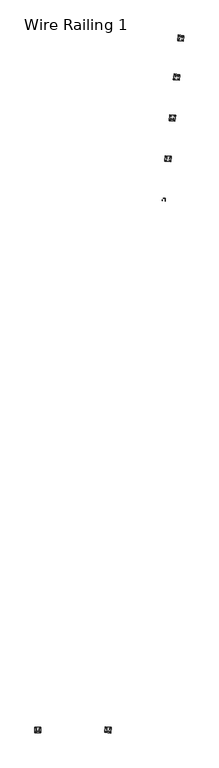
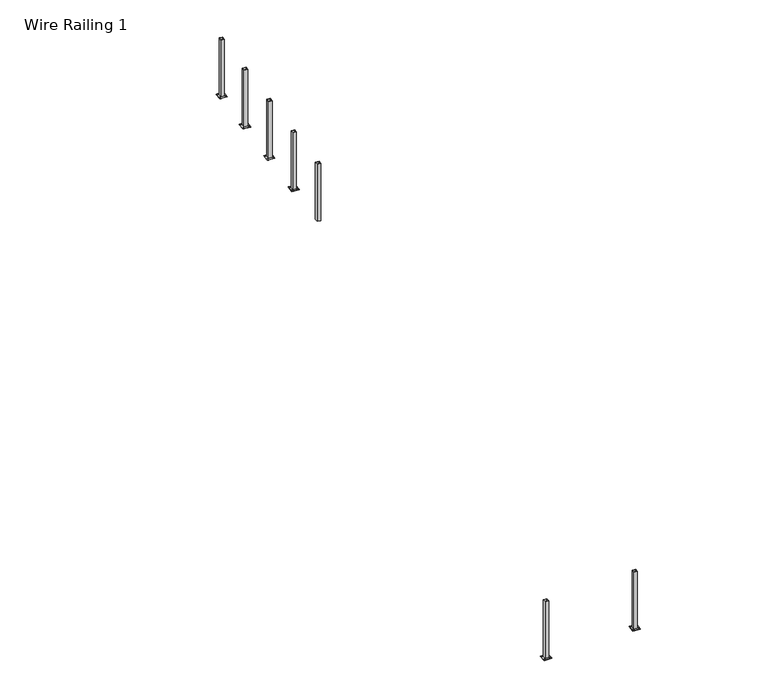
"""IFC4 building model written with IfcOpenShell, lengths in millimetres: railing geometry, Wire Railing 1."""

import ifcopenshell
import ifcopenshell.guid

model = None  # the IFC model being written
_history = None  # IfcOwnerHistory: only IFC2X3 demands one
_inside = {}  # id of a spatial element -> (the spatial element, [elements in it])
_under = {}  # id of a project, library or spatial element -> (it, [spatial elements below it])
_declared = {}  # id of a project -> (the project, [libraries it declares])
_typed = {}  # id of a type object -> (the type object, [elements of that type])
_made_of = {}  # id of a material, layer set ... -> (it, [elements and type objects made of it])


def new_model(schema):
    """Start an empty IFC model of exactly this schema.

    Asked for "IFC4X3", IfcOpenShell would pick the latest addendum, in which some entities
    have other attributes; the version numbers below select the first issue.
    IFC2X3 requires an IfcOwnerHistory on every rooted entity: one is made here for all.
    """
    global model, _history
    if schema == "IFC4X3":
        model = ifcopenshell.file(schema_version=(4, 3, 0, 0))
    else:
        model = ifcopenshell.file(schema=schema)
    _inside.clear()
    _under.clear()
    _declared.clear()
    _typed.clear()
    _made_of.clear()
    _history = None
    if model.schema == "IFC2X3":
        org = make("IfcOrganization", Name="unknown")
        user = make(
            "IfcPersonAndOrganization",
            ThePerson=make("IfcPerson", FamilyName="unknown"),
            TheOrganization=org,
        )
        app = make(
            "IfcApplication",
            ApplicationDeveloper=org,
            Version="unknown",
            ApplicationFullName="unknown",
            ApplicationIdentifier="unknown",
        )
        _history = make(
            "IfcOwnerHistory",
            OwningUser=user,
            OwningApplication=app,
            ChangeAction="ADDED",
            CreationDate=0,
        )
    return model


def make(cls, **values):
    """One entity of the class cls with the attributes given. An attribute that is None is left unset."""
    return model.create_entity(
        cls, **{name: value for name, value in values.items() if value is not None}
    )


def rooted(cls, **values):
    """An entity with a GlobalId (a new one), such as an element, a storey or a relation."""
    return make(cls, GlobalId=ifcopenshell.guid.new(), OwnerHistory=_history, **values)


def si_unit(unit_type, name, prefix=None):
    """IfcSIUnit, for example si_unit("LENGTHUNIT", "METRE", prefix="MILLI")."""
    return make("IfcSIUnit", UnitType=unit_type, Prefix=prefix, Name=name)


def assignment(units):
    """IfcUnitAssignment: the units of a project."""
    return None if units is None else make("IfcUnitAssignment", Units=units)


def point(xyz):
    """IfcCartesianPoint."""
    return None if xyz is None else make("IfcCartesianPoint", Coordinates=xyz)


def direction(xyz):
    """IfcDirection."""
    return None if xyz is None else make("IfcDirection", DirectionRatios=xyz)


def frame(location, z_axis=None, x_axis=None):
    """IfcAxis2Placement3D, a coordinate frame: its origin and axes. An axis left out is left unset."""
    return make(
        "IfcAxis2Placement3D",
        Location=point(location),
        Axis=direction(z_axis),
        RefDirection=direction(x_axis),
    )


def frame_2d(location, x_axis=None):
    """IfcAxis2Placement2D, a coordinate frame in the plane: its origin and x axis."""
    return make(
        "IfcAxis2Placement2D", Location=point(location), RefDirection=direction(x_axis)
    )


def origin():
    """The frame at (0, 0, 0) with its axes left unset."""
    return frame((0.0, 0.0, 0.0))


def place(relative_to, where):
    """IfcLocalPlacement: puts the frame where relative to a parent placement (None: the world)."""
    return make(
        "IfcLocalPlacement", PlacementRelTo=relative_to, RelativePlacement=where
    )


def context(
    kind, dimensions, precision=None, world=None, true_north=None, identifier=None
):
    """IfcGeometricRepresentationContext, for example the 3D "Model" context."""
    return make(
        "IfcGeometricRepresentationContext",
        ContextIdentifier=identifier,
        ContextType=kind,
        CoordinateSpaceDimension=dimensions,
        Precision=precision,
        WorldCoordinateSystem=world,
        TrueNorth=true_north,
    )


def project(units=None, contexts=None):
    """IfcProject with its units and contexts."""
    return rooted(
        "IfcProject",
        Name="project",
        RepresentationContexts=contexts,
        UnitsInContext=assignment(units),
    )


def spatial(cls, under=None, at=None, **own):
    """A site, building, storey or space (cls), placed at a placement, below another one or the project."""
    s = rooted(cls, ObjectPlacement=at, **own)
    if under is not None:
        _under.setdefault(under.id(), (under, []))[1].append(s)
    return s


def polyline(points):
    """IfcPolyline through the points."""
    return make("IfcPolyline", Points=[point(p) for p in points])


def circle_curve(where, radius):
    """IfcCircle in the frame where."""
    return make("IfcCircle", Position=where, Radius=radius)


def trimmed(basis, trim1, trim2, sense, master):
    """IfcTrimmedCurve: the piece of a basis curve between two trims."""
    return make(
        "IfcTrimmedCurve",
        BasisCurve=basis,
        Trim1=trim1,
        Trim2=trim2,
        SenseAgreement=sense,
        MasterRepresentation=master,
    )


def segment(curve, same_sense, transition):
    """IfcCompositeCurveSegment."""
    return make(
        "IfcCompositeCurveSegment",
        Transition=transition,
        SameSense=same_sense,
        ParentCurve=curve,
    )


def composite_curve(segments, self_intersect=None):
    """IfcCompositeCurve: segments joined end to end."""
    return make("IfcCompositeCurve", Segments=segments, SelfIntersect=self_intersect)


def outline(outer, holes=None, kind="AREA"):
    """IfcArbitraryClosedProfileDef: a profile drawn as a closed curve; with holes, ...WithVoids."""
    if holes is None:
        return make("IfcArbitraryClosedProfileDef", ProfileType=kind, OuterCurve=outer)
    return make(
        "IfcArbitraryProfileDefWithVoids",
        ProfileType=kind,
        OuterCurve=outer,
        InnerCurves=holes,
    )


def extrude(swept, where, along, depth):
    """IfcExtrudedAreaSolid: the profile swept, set in the frame where, extruded along a direction by depth."""
    return make(
        "IfcExtrudedAreaSolid",
        SweptArea=swept,
        Position=where,
        ExtrudedDirection=direction(along),
        Depth=depth,
    )


def shape(context_of_items, identifier, shape_type, items):
    """IfcShapeRepresentation: the items that make up one representation, for example the "Body"."""
    return make(
        "IfcShapeRepresentation",
        ContextOfItems=context_of_items,
        RepresentationIdentifier=identifier,
        RepresentationType=shape_type,
        Items=items,
    )


def source(mapping_origin, context_of_items, identifier, shape_type, items):
    """IfcRepresentationMap: a shape defined once, which mapped items show again and again."""
    return make(
        "IfcRepresentationMap",
        MappingOrigin=mapping_origin,
        MappedRepresentation=shape(context_of_items, identifier, shape_type, items),
    )


def transform(
    local_origin,
    x_axis=None,
    y_axis=None,
    z_axis=None,
    scale=None,
    scale2=None,
    scale3=None,
    uniform=True,
):
    """IfcCartesianTransformationOperator3D, or its non-uniform kind. x_axis, y_axis, z_axis: its Axis1, 2, 3."""
    if uniform:
        return make(
            "IfcCartesianTransformationOperator3D",
            Axis1=direction(x_axis),
            Axis2=direction(y_axis),
            LocalOrigin=point(local_origin),
            Scale=scale,
            Axis3=direction(z_axis),
        )
    return make(
        "IfcCartesianTransformationOperator3DnonUniform",
        Axis1=direction(x_axis),
        Axis2=direction(y_axis),
        LocalOrigin=point(local_origin),
        Scale=scale,
        Axis3=direction(z_axis),
        Scale2=scale2,
        Scale3=scale3,
    )


def mapped(mapping_source, mapping_target):
    """IfcMappedItem: shows the shape of a source again, moved by a transform."""
    return make(
        "IfcMappedItem", MappingSource=mapping_source, MappingTarget=mapping_target
    )


def made_of(thing, what):
    """Note that an element or type object is made of a material, layer set ...; save() writes the relation."""
    if what is not None:
        _made_of.setdefault(what.id(), (what, []))[1].append(thing)
    return thing


def element(
    cls,
    number,
    at=None,
    inside=None,
    cuts=None,
    type_object=None,
    material=None,
    context=None,
    identifier="Body",
    shape_type=None,
    held_by="IfcProductDefinitionShape",
    body=None,
    shapes=None,
    **own,
):
    """One element of the class cls, such as IfcWall. Its Tag is "e" and its number.

    at: its placement. inside: the storey or other place that contains it. cuts: it is an
    opening in that element (IfcRelVoidsElement). A single representation is given by context,
    identifier, shape_type and body (its items); several are given by shapes. held_by: the class
    of the entity that holds the representations. save() writes the other relations.
    """
    e = rooted(cls, Tag="e%d" % number, ObjectPlacement=at, **own)
    if body is not None:
        shapes = [shape(context, identifier, shape_type, body)]
    if shapes is not None:
        e.Representation = make(held_by, Representations=shapes)
    if inside is not None:
        _inside.setdefault(inside.id(), (inside, []))[1].append(e)
    if cuts is not None:
        rooted(
            "IfcRelVoidsElement", RelatingBuildingElement=cuts, RelatedOpeningElement=e
        )
    if type_object is not None:
        _typed.setdefault(type_object.id(), (type_object, []))[1].append(e)
    return made_of(e, material)


def aggregate(whole, parts):
    """IfcRelAggregates: a whole, such as a stair, and the parts it consists of."""
    return rooted("IfcRelAggregates", RelatingObject=whole, RelatedObjects=parts)


def save(model, path):
    """Write the relations noted so far, then the file.

    IfcRelAggregates (storeys below a building ...), IfcRelContainedInSpatialStructure (elements
    in a storey), IfcRelDefinesByType, IfcRelAssociatesMaterial and IfcRelDeclares: one each for
    every whole, place, type object, material and project.
    """
    for whole, parts in _under.values():
        aggregate(whole, parts)
    for where, things in _inside.values():
        rooted(
            "IfcRelContainedInSpatialStructure",
            RelatedElements=things,
            RelatingStructure=where,
        )
    for kind, things in _typed.values():
        rooted("IfcRelDefinesByType", RelatedObjects=things, RelatingType=kind)
    for what, things in _made_of.values():
        rooted("IfcRelAssociatesMaterial", RelatedObjects=things, RelatingMaterial=what)
    for by, libraries in _declared.values():
        rooted("IfcRelDeclares", RelatingContext=by, RelatedDefinitions=libraries)
    model.write(path)


def wire_railing_1_27702b10(model_context):
    return source(origin(), model_context, "Body", "SweptSolid", [
        extrude(outline(polyline([(34921.8552452, 37241.7615038), (34981.8497786, 37235.4558243), (34975.544099, 37175.4612909), (34915.5495657, 37181.7669705), (34921.8552452, 37241.7615038)]), holes=[polyline([(34927.5067035, 37234.782534), (34922.5285355, 37187.4184288), (34969.8926407, 37182.4402607), (34974.8708088, 37229.804366), (34927.5067035, 37234.782534)])]), frame((0.0, 0.0, 266395.2), z_axis=(0.0, 0.0, 1.0), x_axis=(1.0, 0.0, 0.0)), (0.0, 0.0, 1.0), 1047.75),
        extrude(outline(composite_curve([segment(trimmed(circle_curve(frame_2d((35091.5302664, 38142.3107005)), 6.35), [point((35097.8454804, 38141.6469448))], [point((35085.2150524, 38142.9744562))], False, "CARTESIAN"), True, "CONTINUOUS"), segment(trimmed(circle_curve(frame_2d((35091.5302664, 38142.3107005)), 6.35), [point((35085.2150524, 38142.9744562))], [point((35097.8454804, 38141.6469448))], False, "CARTESIAN"), True, "CONTINUOUS")], self_intersect=False)), frame((0.0, 0.0, 266395.2), z_axis=(0.0, 0.0, 1.0), x_axis=(1.0, 0.0, 0.0)), (0.0, 0.0, 1.0), 12.7),
        extrude(outline(composite_curve([segment(trimmed(circle_curve(frame_2d((35003.1172699, 38151.6032809)), 6.35), [point((35009.4324839, 38150.9395251))], [point((34996.8020559, 38152.2670366))], False, "CARTESIAN"), True, "CONTINUOUS"), segment(trimmed(circle_curve(frame_2d((35003.1172699, 38151.6032809)), 6.35), [point((34996.8020559, 38152.2670366))], [point((35009.4324839, 38150.9395251))], False, "CARTESIAN"), True, "CONTINUOUS")], self_intersect=False)), frame((0.0, 0.0, 266395.2), z_axis=(0.0, 0.0, 1.0), x_axis=(1.0, 0.0, 0.0)), (0.0, 0.0, 1.0), 12.7),
        extrude(outline(composite_curve([segment(trimmed(circle_curve(frame_2d((35082.237686, 38053.897704)), 6.35), [point((35088.5529, 38053.2339483))], [point((35075.922472, 38054.5614597))], False, "CARTESIAN"), True, "CONTINUOUS"), segment(trimmed(circle_curve(frame_2d((35082.237686, 38053.897704)), 6.35), [point((35075.922472, 38054.5614597))], [point((35088.5529, 38053.2339483))], False, "CARTESIAN"), True, "CONTINUOUS")], self_intersect=False)), frame((0.0, 0.0, 266395.2), z_axis=(0.0, 0.0, 1.0), x_axis=(1.0, 0.0, 0.0)), (0.0, 0.0, 1.0), 12.7),
        extrude(outline(composite_curve([segment(trimmed(circle_curve(frame_2d((34993.8246895, 38063.1902844)), 6.35), [point((35000.1399035, 38062.5265286))], [point((34987.5094755, 38063.8540401))], False, "CARTESIAN"), True, "CONTINUOUS"), segment(trimmed(circle_curve(frame_2d((34993.8246895, 38063.1902844)), 6.35), [point((34987.5094755, 38063.8540401))], [point((35000.1399035, 38062.5265286))], False, "CARTESIAN"), True, "CONTINUOUS")], self_intersect=False)), frame((0.0, 0.0, 266395.2), z_axis=(0.0, 0.0, 1.0), x_axis=(1.0, 0.0, 0.0)), (0.0, 0.0, 1.0), 12.7),
        extrude(outline(polyline([(34986.162895, 38172.5401902), (35112.4671757, 38159.2650754), (35099.1920609, 38032.9607947), (34972.8877802, 38046.2359095), (34986.162895, 38172.5401902)])), frame((0.0, 0.0, 266395.2), z_axis=(0.0, 0.0, 1.0), x_axis=(1.0, 0.0, 0.0)), (0.0, 0.0, 1.0), 6.35),
        extrude(outline(polyline([(35015.8330511, 38135.9005989), (35075.8275844, 38129.5949193), (35069.5219049, 38069.600386), (35009.5273715, 38075.9060655), (35015.8330511, 38135.9005989)]), holes=[polyline([(35021.4845094, 38128.9216291), (35016.5063413, 38081.5575238), (35063.8704466, 38076.5793558), (35068.8486146, 38123.943461), (35021.4845094, 38128.9216291)])]), frame((0.0, 0.0, 266395.2), z_axis=(0.0, 0.0, 1.0), x_axis=(1.0, 0.0, 0.0)), (0.0, 0.0, 1.0), 1047.75),
        extrude(outline(composite_curve([segment(trimmed(circle_curve(frame_2d((35185.5080722, 39036.4497956)), 6.35), [point((35191.8232862, 39035.7860398))], [point((35179.1928582, 39037.1135513))], False, "CARTESIAN"), True, "CONTINUOUS"), segment(trimmed(circle_curve(frame_2d((35185.5080722, 39036.4497956)), 6.35), [point((35179.1928582, 39037.1135513))], [point((35191.8232862, 39035.7860398))], False, "CARTESIAN"), True, "CONTINUOUS")], self_intersect=False)), frame((0.0, 0.0, 266395.2), z_axis=(0.0, 0.0, 1.0), x_axis=(1.0, 0.0, 0.0)), (0.0, 0.0, 1.0), 12.7),
        extrude(outline(composite_curve([segment(trimmed(circle_curve(frame_2d((35097.0950757, 39045.742376)), 6.35), [point((35103.4102897, 39045.0786202))], [point((35090.7798617, 39046.4061317))], False, "CARTESIAN"), True, "CONTINUOUS"), segment(trimmed(circle_curve(frame_2d((35097.0950757, 39045.742376)), 6.35), [point((35090.7798617, 39046.4061317))], [point((35103.4102897, 39045.0786202))], False, "CARTESIAN"), True, "CONTINUOUS")], self_intersect=False)), frame((0.0, 0.0, 266395.2), z_axis=(0.0, 0.0, 1.0), x_axis=(1.0, 0.0, 0.0)), (0.0, 0.0, 1.0), 12.7),
        extrude(outline(composite_curve([segment(trimmed(circle_curve(frame_2d((35176.2154918, 38948.0367991)), 6.35), [point((35182.5307059, 38947.3730434))], [point((35169.9002778, 38948.7005548))], False, "CARTESIAN"), True, "CONTINUOUS"), segment(trimmed(circle_curve(frame_2d((35176.2154918, 38948.0367991)), 6.35), [point((35169.9002778, 38948.7005548))], [point((35182.5307059, 38947.3730434))], False, "CARTESIAN"), True, "CONTINUOUS")], self_intersect=False)), frame((0.0, 0.0, 266395.2), z_axis=(0.0, 0.0, 1.0), x_axis=(1.0, 0.0, 0.0)), (0.0, 0.0, 1.0), 12.7),
        extrude(outline(composite_curve([segment(trimmed(circle_curve(frame_2d((35087.8024953, 38957.3293795)), 6.35), [point((35094.1177094, 38956.6656237))], [point((35081.4872813, 38957.9931352))], False, "CARTESIAN"), True, "CONTINUOUS"), segment(trimmed(circle_curve(frame_2d((35087.8024953, 38957.3293795)), 6.35), [point((35081.4872813, 38957.9931352))], [point((35094.1177094, 38956.6656237))], False, "CARTESIAN"), True, "CONTINUOUS")], self_intersect=False)), frame((0.0, 0.0, 266395.2), z_axis=(0.0, 0.0, 1.0), x_axis=(1.0, 0.0, 0.0)), (0.0, 0.0, 1.0), 12.7),
        extrude(outline(polyline([(35080.1407008, 39066.6792853), (35206.4449815, 39053.4041705), (35193.1698667, 38927.0998898), (35066.865586, 38940.3750046), (35080.1407008, 39066.6792853)])), frame((0.0, 0.0, 266395.2), z_axis=(0.0, 0.0, 1.0), x_axis=(1.0, 0.0, 0.0)), (0.0, 0.0, 1.0), 6.35),
        extrude(outline(polyline([(35109.8108569, 39030.039694), (35169.8053902, 39023.7340144), (35163.4997107, 38963.7394811), (35103.5051773, 38970.0451606), (35109.8108569, 39030.039694)]), holes=[polyline([(35115.4623152, 39023.0607242), (35110.4841471, 38975.6966189), (35157.8482524, 38970.7184509), (35162.8264204, 39018.0825561), (35115.4623152, 39023.0607242)])]), frame((0.0, 0.0, 266395.2), z_axis=(0.0, 0.0, 1.0), x_axis=(1.0, 0.0, 0.0)), (0.0, 0.0, 1.0), 1047.75),
        extrude(outline(composite_curve([segment(trimmed(circle_curve(frame_2d((35279.485878, 39930.5888907)), 6.35), [point((35285.8010921, 39929.9251349))], [point((35273.170664, 39931.2526464))], False, "CARTESIAN"), True, "CONTINUOUS"), segment(trimmed(circle_curve(frame_2d((35279.485878, 39930.5888907)), 6.35), [point((35273.170664, 39931.2526464))], [point((35285.8010921, 39929.9251349))], False, "CARTESIAN"), True, "CONTINUOUS")], self_intersect=False)), frame((0.0, 0.0, 266395.2), z_axis=(0.0, 0.0, 1.0), x_axis=(1.0, 0.0, 0.0)), (0.0, 0.0, 1.0), 12.7),
        extrude(outline(composite_curve([segment(trimmed(circle_curve(frame_2d((35191.0728815, 39939.8814711)), 6.35), [point((35197.3880956, 39939.2177153))], [point((35184.7576675, 39940.5452268))], False, "CARTESIAN"), True, "CONTINUOUS"), segment(trimmed(circle_curve(frame_2d((35191.0728815, 39939.8814711)), 6.35), [point((35184.7576675, 39940.5452268))], [point((35197.3880956, 39939.2177153))], False, "CARTESIAN"), True, "CONTINUOUS")], self_intersect=False)), frame((0.0, 0.0, 266395.2), z_axis=(0.0, 0.0, 1.0), x_axis=(1.0, 0.0, 0.0)), (0.0, 0.0, 1.0), 12.7),
        extrude(outline(composite_curve([segment(trimmed(circle_curve(frame_2d((35270.1932976, 39842.1758942)), 6.35), [point((35276.5085117, 39841.5121384))], [point((35263.8780836, 39842.8396499))], False, "CARTESIAN"), True, "CONTINUOUS"), segment(trimmed(circle_curve(frame_2d((35270.1932976, 39842.1758942)), 6.35), [point((35263.8780836, 39842.8396499))], [point((35276.5085117, 39841.5121384))], False, "CARTESIAN"), True, "CONTINUOUS")], self_intersect=False)), frame((0.0, 0.0, 266395.2), z_axis=(0.0, 0.0, 1.0), x_axis=(1.0, 0.0, 0.0)), (0.0, 0.0, 1.0), 12.7),
        extrude(outline(composite_curve([segment(trimmed(circle_curve(frame_2d((35181.7803011, 39851.4684746)), 6.35), [point((35188.0955152, 39850.8047188))], [point((35175.4650871, 39852.1322303))], False, "CARTESIAN"), True, "CONTINUOUS"), segment(trimmed(circle_curve(frame_2d((35181.7803011, 39851.4684746)), 6.35), [point((35175.4650871, 39852.1322303))], [point((35188.0955152, 39850.8047188))], False, "CARTESIAN"), True, "CONTINUOUS")], self_intersect=False)), frame((0.0, 0.0, 266395.2), z_axis=(0.0, 0.0, 1.0), x_axis=(1.0, 0.0, 0.0)), (0.0, 0.0, 1.0), 12.7),
        extrude(outline(polyline([(35174.1185066, 39960.8183804), (35300.4227873, 39947.5432656), (35287.1476725, 39821.2389849), (35160.8433918, 39834.5140997), (35174.1185066, 39960.8183804)])), frame((0.0, 0.0, 266395.2), z_axis=(0.0, 0.0, 1.0), x_axis=(1.0, 0.0, 0.0)), (0.0, 0.0, 1.0), 6.35),
        extrude(outline(polyline([(35203.7886627, 39924.1787891), (35263.783196, 39917.8731095), (35257.4775165, 39857.8785762), (35197.4829831, 39864.1842557), (35203.7886627, 39924.1787891)]), holes=[polyline([(35209.440121, 39917.1998193), (35204.4619529, 39869.835714), (35251.8260582, 39864.857546), (35256.8042262, 39912.2216512), (35209.440121, 39917.1998193)])]), frame((0.0, 0.0, 266395.2), z_axis=(0.0, 0.0, 1.0), x_axis=(1.0, 0.0, 0.0)), (0.0, 0.0, 1.0), 1047.75),
        extrude(outline(composite_curve([segment(trimmed(circle_curve(frame_2d((33775.840985, 25624.3633693)), 6.35), [point((33782.1561991, 25623.6996135))], [point((33769.525771, 25625.027125))], False, "CARTESIAN"), True, "CONTINUOUS"), segment(trimmed(circle_curve(frame_2d((33775.840985, 25624.3633693)), 6.35), [point((33769.525771, 25625.027125))], [point((33782.1561991, 25623.6996135))], False, "CARTESIAN"), True, "CONTINUOUS")], self_intersect=False)), frame((0.0, 0.0, 266395.2), z_axis=(0.0, 0.0, 1.0), x_axis=(1.0, 0.0, 0.0)), (0.0, 0.0, 1.0), 12.7),
        extrude(outline(composite_curve([segment(trimmed(circle_curve(frame_2d((33687.4279886, 25633.6559496)), 6.35), [point((33693.7432026, 25632.9921939))], [point((33681.1127745, 25634.3197054))], False, "CARTESIAN"), True, "CONTINUOUS"), segment(trimmed(circle_curve(frame_2d((33687.4279886, 25633.6559496)), 6.35), [point((33681.1127745, 25634.3197054))], [point((33693.7432026, 25632.9921939))], False, "CARTESIAN"), True, "CONTINUOUS")], self_intersect=False)), frame((0.0, 0.0, 266395.2), z_axis=(0.0, 0.0, 1.0), x_axis=(1.0, 0.0, 0.0)), (0.0, 0.0, 1.0), 12.7),
        extrude(outline(composite_curve([segment(trimmed(circle_curve(frame_2d((33766.5484047, 25535.9503728)), 6.35), [point((33772.8636187, 25535.286617))], [point((33760.2331906, 25536.6141285))], False, "CARTESIAN"), True, "CONTINUOUS"), segment(trimmed(circle_curve(frame_2d((33766.5484047, 25535.9503728)), 6.35), [point((33760.2331906, 25536.6141285))], [point((33772.8636187, 25535.286617))], False, "CARTESIAN"), True, "CONTINUOUS")], self_intersect=False)), frame((0.0, 0.0, 266395.2), z_axis=(0.0, 0.0, 1.0), x_axis=(1.0, 0.0, 0.0)), (0.0, 0.0, 1.0), 12.7),
        extrude(outline(composite_curve([segment(trimmed(circle_curve(frame_2d((33678.1354082, 25545.2429531)), 6.35), [point((33684.4506222, 25544.5791974))], [point((33671.8201941, 25545.9067089))], False, "CARTESIAN"), True, "CONTINUOUS"), segment(trimmed(circle_curve(frame_2d((33678.1354082, 25545.2429531)), 6.35), [point((33671.8201941, 25545.9067089))], [point((33684.4506222, 25544.5791974))], False, "CARTESIAN"), True, "CONTINUOUS")], self_intersect=False)), frame((0.0, 0.0, 266395.2), z_axis=(0.0, 0.0, 1.0), x_axis=(1.0, 0.0, 0.0)), (0.0, 0.0, 1.0), 12.7),
        extrude(outline(polyline([(33670.4736137, 25654.592859), (33796.7778944, 25641.3177441), (33783.5027795, 25515.0134634), (33657.1984988, 25528.2885783), (33670.4736137, 25654.592859)])), frame((0.0, 0.0, 266395.2), z_axis=(0.0, 0.0, 1.0), x_axis=(1.0, 0.0, 0.0)), (0.0, 0.0, 1.0), 6.35),
        extrude(outline(polyline([(33700.1437697, 25617.9532676), (33760.1383031, 25611.6475881), (33753.8326235, 25551.6530548), (33693.8380902, 25557.9587343), (33700.1437697, 25617.9532676)]), holes=[polyline([(33705.795228, 25610.9742979), (33700.8170599, 25563.6101926), (33748.1811652, 25558.6320245), (33753.1593333, 25605.9961298), (33705.795228, 25610.9742979)])]), frame((0.0, 0.0, 266395.2), z_axis=(0.0, 0.0, 1.0), x_axis=(1.0, 0.0, 0.0)), (0.0, 0.0, 1.0), 1047.75),
        extrude(outline(composite_curve([segment(trimmed(circle_curve(frame_2d((32231.9590378, 25540.3531612)), 6.35), [point((32231.9590378, 25534.0031612))], [point((32231.9590378, 25546.7031612))], False, "CARTESIAN"), True, "CONTINUOUS"), segment(trimmed(circle_curve(frame_2d((32231.9590378, 25540.3531612)), 6.35), [point((32231.9590378, 25546.7031612))], [point((32231.9590378, 25534.0031612))], False, "CARTESIAN"), True, "CONTINUOUS")], self_intersect=False)), frame((0.0, 0.0, 266395.2), z_axis=(0.0, 0.0, 1.0), x_axis=(1.0, 0.0, 0.0)), (0.0, 0.0, 1.0), 12.7),
        extrude(outline(composite_curve([segment(trimmed(circle_curve(frame_2d((32231.9590378, 25629.2531612)), 6.35), [point((32231.9590378, 25622.9031612))], [point((32231.9590378, 25635.6031612))], False, "CARTESIAN"), True, "CONTINUOUS"), segment(trimmed(circle_curve(frame_2d((32231.9590378, 25629.2531612)), 6.35), [point((32231.9590378, 25635.6031612))], [point((32231.9590378, 25622.9031612))], False, "CARTESIAN"), True, "CONTINUOUS")], self_intersect=False)), frame((0.0, 0.0, 266395.2), z_axis=(0.0, 0.0, 1.0), x_axis=(1.0, 0.0, 0.0)), (0.0, 0.0, 1.0), 12.7),
        extrude(outline(composite_curve([segment(trimmed(circle_curve(frame_2d((32143.0590378, 25540.3531612)), 6.35), [point((32143.0590378, 25534.0031612))], [point((32143.0590378, 25546.7031612))], False, "CARTESIAN"), True, "CONTINUOUS"), segment(trimmed(circle_curve(frame_2d((32143.0590378, 25540.3531612)), 6.35), [point((32143.0590378, 25546.7031612))], [point((32143.0590378, 25534.0031612))], False, "CARTESIAN"), True, "CONTINUOUS")], self_intersect=False)), frame((0.0, 0.0, 266395.2), z_axis=(0.0, 0.0, 1.0), x_axis=(1.0, 0.0, 0.0)), (0.0, 0.0, 1.0), 12.7),
        extrude(outline(composite_curve([segment(trimmed(circle_curve(frame_2d((32143.0590378, 25629.2531612)), 6.35), [point((32143.0590378, 25622.9031612))], [point((32143.0590378, 25635.6031612))], False, "CARTESIAN"), True, "CONTINUOUS"), segment(trimmed(circle_curve(frame_2d((32143.0590378, 25629.2531612)), 6.35), [point((32143.0590378, 25635.6031612))], [point((32143.0590378, 25622.9031612))], False, "CARTESIAN"), True, "CONTINUOUS")], self_intersect=False)), frame((0.0, 0.0, 266395.2), z_axis=(0.0, 0.0, 1.0), x_axis=(1.0, 0.0, 0.0)), (0.0, 0.0, 1.0), 12.7),
        extrude(outline(polyline([(32251.0090378, 25648.3031612), (32251.0090378, 25521.3031612), (32124.0090378, 25521.3031612), (32124.0090378, 25648.3031612), (32251.0090378, 25648.3031612)])), frame((0.0, 0.0, 266395.2), z_axis=(0.0, 0.0, 1.0), x_axis=(1.0, 0.0, 0.0)), (0.0, 0.0, 1.0), 6.35),
        extrude(outline(polyline([(32217.6715378, 25614.9656612), (32217.6715378, 25554.6406612), (32157.3465378, 25554.6406612), (32157.3465378, 25614.9656612), (32217.6715378, 25614.9656612)]), holes=[polyline([(32211.3215378, 25608.6156612), (32163.6965378, 25608.6156612), (32163.6965378, 25560.9906612), (32211.3215378, 25560.9906612), (32211.3215378, 25608.6156612)])]), frame((0.0, 0.0, 266395.2), z_axis=(0.0, 0.0, 1.0), x_axis=(1.0, 0.0, 0.0)), (0.0, 0.0, 1.0), 1047.75),
        extrude(outline(composite_curve([segment(trimmed(circle_curve(frame_2d((35369.4811494, 40786.8367016)), 6.35), [point((35375.7963634, 40786.1729458))], [point((35363.1659353, 40787.5004573))], False, "CARTESIAN"), True, "CONTINUOUS"), segment(trimmed(circle_curve(frame_2d((35369.4811494, 40786.8367016)), 6.35), [point((35363.1659353, 40787.5004573))], [point((35375.7963634, 40786.1729458))], False, "CARTESIAN"), True, "CONTINUOUS")], self_intersect=False)), frame((0.0, 0.0, 266395.2), z_axis=(0.0, 0.0, 1.0), x_axis=(1.0, 0.0, 0.0)), (0.0, 0.0, 1.0), 12.7),
        extrude(outline(composite_curve([segment(trimmed(circle_curve(frame_2d((35281.0681529, 40796.1292819)), 6.35), [point((35287.3833669, 40795.4655262))], [point((35274.7529388, 40796.7930377))], False, "CARTESIAN"), True, "CONTINUOUS"), segment(trimmed(circle_curve(frame_2d((35281.0681529, 40796.1292819)), 6.35), [point((35274.7529388, 40796.7930377))], [point((35287.3833669, 40795.4655262))], False, "CARTESIAN"), True, "CONTINUOUS")], self_intersect=False)), frame((0.0, 0.0, 266395.2), z_axis=(0.0, 0.0, 1.0), x_axis=(1.0, 0.0, 0.0)), (0.0, 0.0, 1.0), 12.7),
        extrude(outline(composite_curve([segment(trimmed(circle_curve(frame_2d((35360.188569, 40698.4237051)), 6.35), [point((35366.503783, 40697.7599493))], [point((35353.873355, 40699.0874608))], False, "CARTESIAN"), True, "CONTINUOUS"), segment(trimmed(circle_curve(frame_2d((35360.188569, 40698.4237051)), 6.35), [point((35353.873355, 40699.0874608))], [point((35366.503783, 40697.7599493))], False, "CARTESIAN"), True, "CONTINUOUS")], self_intersect=False)), frame((0.0, 0.0, 266395.2), z_axis=(0.0, 0.0, 1.0), x_axis=(1.0, 0.0, 0.0)), (0.0, 0.0, 1.0), 12.7),
        extrude(outline(composite_curve([segment(trimmed(circle_curve(frame_2d((35271.7755725, 40707.7162854)), 6.35), [point((35278.0907865, 40707.0525297))], [point((35265.4603585, 40708.3800412))], False, "CARTESIAN"), True, "CONTINUOUS"), segment(trimmed(circle_curve(frame_2d((35271.7755725, 40707.7162854)), 6.35), [point((35265.4603585, 40708.3800412))], [point((35278.0907865, 40707.0525297))], False, "CARTESIAN"), True, "CONTINUOUS")], self_intersect=False)), frame((0.0, 0.0, 266395.2), z_axis=(0.0, 0.0, 1.0), x_axis=(1.0, 0.0, 0.0)), (0.0, 0.0, 1.0), 12.7),
        extrude(outline(polyline([(35264.113778, 40817.0661913), (35390.4180587, 40803.7910764), (35377.1429439, 40677.4867957), (35250.8386632, 40690.7619106), (35264.113778, 40817.0661913)])), frame((0.0, 0.0, 266395.2), z_axis=(0.0, 0.0, 1.0), x_axis=(1.0, 0.0, 0.0)), (0.0, 0.0, 1.0), 6.35),
        extrude(outline(polyline([(35293.783934, 40780.4265999), (35353.7784674, 40774.1209204), (35347.4727878, 40714.1263871), (35287.4782545, 40720.4320666), (35293.783934, 40780.4265999)]), holes=[polyline([(35299.4353923, 40773.4476302), (35294.4572243, 40726.0835249), (35341.8213295, 40721.1053568), (35346.7994976, 40768.4694621), (35299.4353923, 40773.4476302)])]), frame((0.0, 0.0, 266395.2), z_axis=(0.0, 0.0, 1.0), x_axis=(1.0, 0.0, 0.0)), (0.0, 0.0, 1.0), 1047.75),
    ])


if __name__ == "__main__":
    model = new_model("IFC4")
    model_context = context("Model", 3, world=origin())
    ifc_project = project(units=[si_unit("LENGTHUNIT", "METRE", prefix="MILLI")], contexts=[model_context])
    site = spatial("IfcSite", under=ifc_project)
    building = spatial("IfcBuilding", under=site)
    placement = place(None, origin())
    wire_railing_1_shape = wire_railing_1_27702b10(model_context)
    element("IfcRailing", 1, ObjectType="Wire Railing 1", at=placement, inside=building, context=model_context, shape_type="MappedRepresentation", body=[
        mapped(wire_railing_1_shape, transform((0.0, 0.0, 0.0), x_axis=(1.0, 0.0, 0.0), y_axis=(0.0, 1.0, 0.0), z_axis=(0.0, 0.0, 1.0))),
    ])
    save(model, "model.ifc")

# Revit data of these elements
# Element 1 (IfcRailing, "Wire Railing 1")
#   Materials on its faces: "WIRE RAILING"
# Materials
#   "WIRE RAILING": class "Metal", colour RGB 244 244 244, transparency 0, Manufacturer = "Kawneer", URL = "http://www.kawneer.com/kawneer/north_america/en/home.asp", Cost = 0
